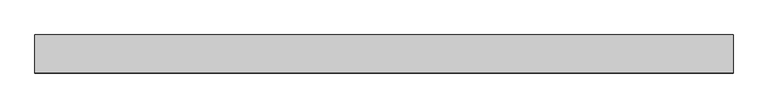
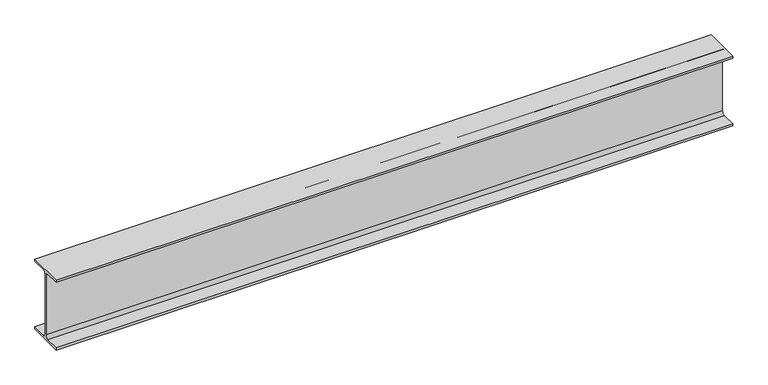
"""IFC4 building model written with IfcOpenShell, lengths in millimetres: beam geometry, Steel Framing_H_KS : H_SB_AR_S02_H-300x150x6.5x9_WG1."""

from ifc_helpers import new_model, si_unit, point, frame, frame_2d, origin, place, context, project, spatial, polyline, circle_curve, trimmed, segment, composite_curve, outline, extrude, source, transform, mapped, element, save


def beam_c8dce8fe(model_context):
    return source(origin(), model_context, "Body", "SweptSolid", [
        extrude(outline(composite_curve([segment(polyline([(-75.0, -141.0), (-16.25, -141.0)]), True, "CONTINUOUS"), segment(trimmed(circle_curve(frame_2d((-16.25, -128.0)), 13.0), [point((-16.25, -141.0))], [point((-3.25, -128.0))], True, "CARTESIAN"), True, "CONTINUOUS"), segment(polyline([(-3.25, -128.0), (-3.25, 128.0)]), True, "CONTINUOUS"), segment(trimmed(circle_curve(frame_2d((-16.25, 128.0)), 13.0), [point((-3.25, 128.0))], [point((-16.25, 141.0))], True, "CARTESIAN"), True, "CONTINUOUS"), segment(polyline([(-16.25, 141.0), (-75.0, 141.0), (-75.0, 150.0), (75.0, 150.0), (75.0, 141.0), (16.25, 141.0)]), True, "CONTINUOUS"), segment(trimmed(circle_curve(frame_2d((16.25, 128.0)), 13.0), [point((16.25, 141.0))], [point((3.25, 128.0))], True, "CARTESIAN"), True, "CONTINUOUS"), segment(polyline([(3.25, 128.0), (3.25, -128.0)]), True, "CONTINUOUS"), segment(trimmed(circle_curve(frame_2d((16.25, -128.0)), 13.0), [point((3.25, -128.0))], [point((16.25, -141.0))], True, "CARTESIAN"), True, "CONTINUOUS"), segment(polyline([(16.25, -141.0), (75.0, -141.0), (75.0, -150.0), (-75.0, -150.0), (-75.0, -141.0)]), True, "CONTINUOUS")], self_intersect=False)), frame((-1337.3, 0.0, 0.0), z_axis=(1.0, 0.0, 0.0), x_axis=(0.0, 1.0, 0.0)), (0.0, 0.0, 1.0), 2749.6),
    ])


if __name__ == "__main__":
    model = new_model("IFC4")
    model_context = context("Model", 3, world=origin())
    ifc_project = project(units=[si_unit("LENGTHUNIT", "METRE", prefix="MILLI")], contexts=[model_context])
    site = spatial("IfcSite", under=ifc_project)
    building = spatial("IfcBuilding", under=site)
    placement = place(None, origin())
    beam_shape = beam_c8dce8fe(model_context)
    element("IfcBeam", 1, ObjectType="Steel Framing_H_KS : H_SB_AR_S02_H-300x150x6.5x9_WG1", at=placement, inside=building, context=model_context, shape_type="MappedRepresentation", body=[
        mapped(beam_shape, transform((0.0, 0.0, 0.0), x_axis=(1.0, 0.0, 0.0), y_axis=(0.0, 1.0, 0.0), z_axis=(0.0, 0.0, 1.0))),
    ])
    save(model, "model.ifc")

# Revit data of these elements
# Type "Steel Framing_H_KS : H_SB_AR_S02_H-300x150x6.5x9_WG1"
#   Type Comments = "MAIN"
#   Type Mark = "WG1"
#   H_SectionID = "H-300x150x6.5x9"
#   H_Ratio for Additional Steel Plate = 0.2
#   Width = 15.0 cm
#   Web Thickness = 0.65 cm
#   Web Fillet = 1.3 cm
#   Warping Constant = 107000.0 cm⁶
#   Torsional Moment of Inertia = 9.9539 cm⁴
#   Section Area = 46.78 cm²
#   Plastic Modulus weak axis = 105.0 cm³
#   Plastic Modulus strong axis = 542.0 cm³
#   Perimeter = 1.17 m²/m
#   Nominal Weight = 36.70 kgf/m
#   Moment of Inertia weak axis = 508.00 cm⁴
#   Moment of Inertia strong axis = 7210.00 cm⁴
#   Height = 30.0 cm
#   Flange Thickness = 0.9 cm
#   Elastic Modulus weak axis = 67.7 cm³
#   Elastic Modulus strong axis = 481.0 cm³
#   Centroid Vertical = 15.0 cm
#   Centroid Horizontal = 7.5 cm
#   Bolt Spacing = 8.89 cm
#   Length [instance default] = 1500 mm
#   Structural Material [instance default] = Steel, 45-345
#   Section Name Key = ""
#   Assembly Code = ""
# Element 1 (IfcBeam, "Steel Framing_H_KS : H_SB_AR_S02_H-300x150x6.5x9_WG1")
#   Materials on its faces: "Steel, 45-345"
# Materials
#   "Steel, 45-345": class "Metal", colour RGB 189 187 185, transparency 0, Description = "Steel 345 MPa", Cost = 0
